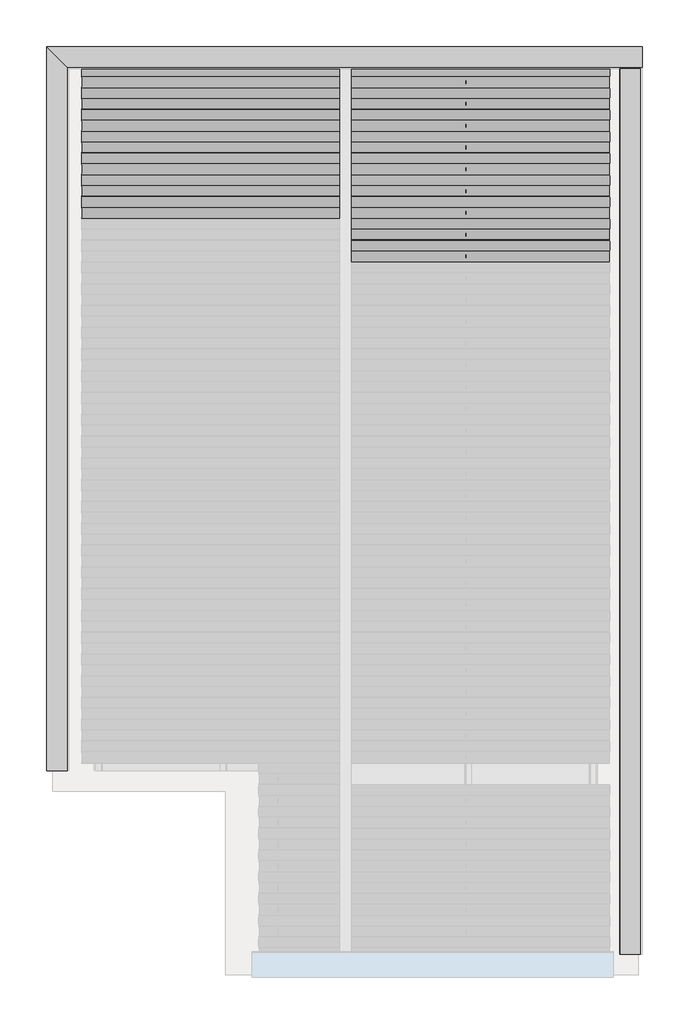
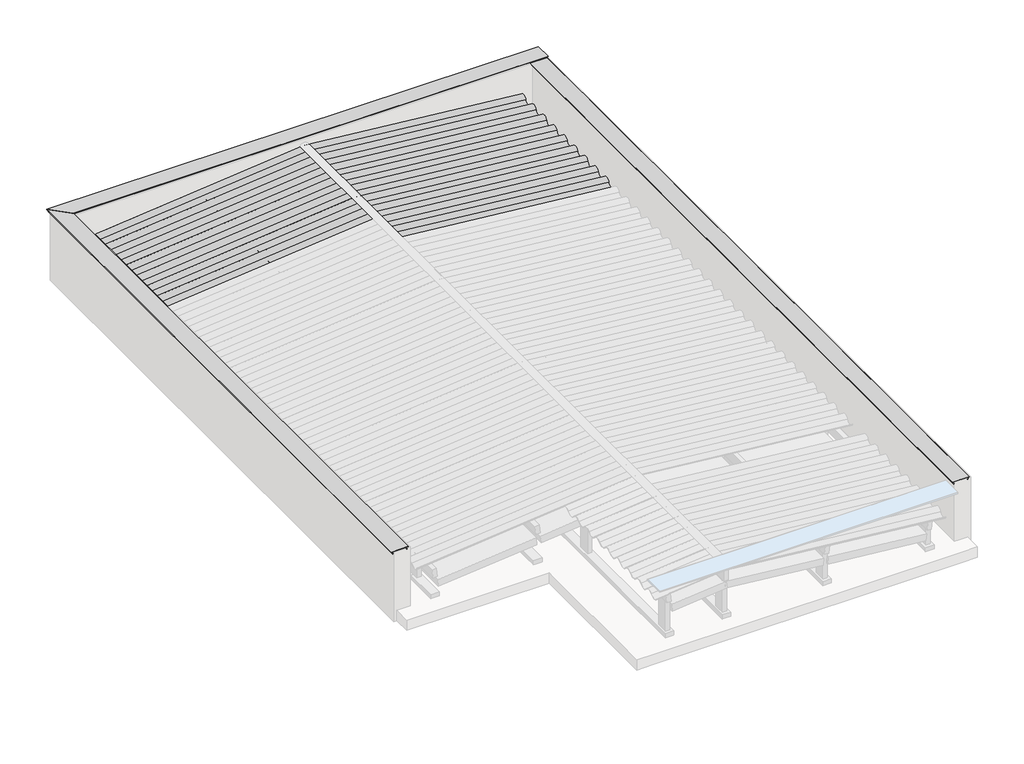
# One storey, part 4 of 4: 23 beams, 10 columns, 1 proxy.
"""IFC4 building model written with IfcOpenShell, lengths in millimetres."""

import ifcopenshell
import ifcopenshell.guid

model = None  # the IFC model being written
_history = None  # IfcOwnerHistory: only IFC2X3 demands one
_inside = {}  # id of a spatial element -> (the spatial element, [elements in it])
_under = {}  # id of a project, library or spatial element -> (it, [spatial elements below it])
_declared = {}  # id of a project -> (the project, [libraries it declares])
_typed = {}  # id of a type object -> (the type object, [elements of that type])
_made_of = {}  # id of a material, layer set ... -> (it, [elements and type objects made of it])


def new_model(schema):
    """Start an empty IFC model of exactly this schema.

    Asked for "IFC4X3", IfcOpenShell would pick the latest addendum, in which some entities
    have other attributes; the version numbers below select the first issue.
    IFC2X3 requires an IfcOwnerHistory on every rooted entity: one is made here for all.
    """
    global model, _history
    if schema == "IFC4X3":
        model = ifcopenshell.file(schema_version=(4, 3, 0, 0))
    else:
        model = ifcopenshell.file(schema=schema)
    _inside.clear()
    _under.clear()
    _declared.clear()
    _typed.clear()
    _made_of.clear()
    _history = None
    if model.schema == "IFC2X3":
        org = make("IfcOrganization", Name="unknown")
        user = make(
            "IfcPersonAndOrganization",
            ThePerson=make("IfcPerson", FamilyName="unknown"),
            TheOrganization=org,
        )
        app = make(
            "IfcApplication",
            ApplicationDeveloper=org,
            Version="unknown",
            ApplicationFullName="unknown",
            ApplicationIdentifier="unknown",
        )
        _history = make(
            "IfcOwnerHistory",
            OwningUser=user,
            OwningApplication=app,
            ChangeAction="ADDED",
            CreationDate=0,
        )
    return model


def make(cls, **values):
    """One entity of the class cls with the attributes given. An attribute that is None is left unset."""
    return model.create_entity(
        cls, **{name: value for name, value in values.items() if value is not None}
    )


def rooted(cls, **values):
    """An entity with a GlobalId (a new one), such as an element, a storey or a relation."""
    return make(cls, GlobalId=ifcopenshell.guid.new(), OwnerHistory=_history, **values)


def si_unit(unit_type, name, prefix=None):
    """IfcSIUnit, for example si_unit("LENGTHUNIT", "METRE", prefix="MILLI")."""
    return make("IfcSIUnit", UnitType=unit_type, Prefix=prefix, Name=name)


def assignment(units):
    """IfcUnitAssignment: the units of a project."""
    return None if units is None else make("IfcUnitAssignment", Units=units)


def point(xyz):
    """IfcCartesianPoint."""
    return None if xyz is None else make("IfcCartesianPoint", Coordinates=xyz)


def direction(xyz):
    """IfcDirection."""
    return None if xyz is None else make("IfcDirection", DirectionRatios=xyz)


def frame(location, z_axis=None, x_axis=None):
    """IfcAxis2Placement3D, a coordinate frame: its origin and axes. An axis left out is left unset."""
    return make(
        "IfcAxis2Placement3D",
        Location=point(location),
        Axis=direction(z_axis),
        RefDirection=direction(x_axis),
    )


def frame_2d(location, x_axis=None):
    """IfcAxis2Placement2D, a coordinate frame in the plane: its origin and x axis."""
    return make(
        "IfcAxis2Placement2D", Location=point(location), RefDirection=direction(x_axis)
    )


def origin():
    """The frame at (0, 0, 0) with its axes left unset."""
    return frame((0.0, 0.0, 0.0))


def place(relative_to, where):
    """IfcLocalPlacement: puts the frame where relative to a parent placement (None: the world)."""
    return make(
        "IfcLocalPlacement", PlacementRelTo=relative_to, RelativePlacement=where
    )


def context(
    kind, dimensions, precision=None, world=None, true_north=None, identifier=None
):
    """IfcGeometricRepresentationContext, for example the 3D "Model" context."""
    return make(
        "IfcGeometricRepresentationContext",
        ContextIdentifier=identifier,
        ContextType=kind,
        CoordinateSpaceDimension=dimensions,
        Precision=precision,
        WorldCoordinateSystem=world,
        TrueNorth=true_north,
    )


def project(units=None, contexts=None):
    """IfcProject with its units and contexts."""
    return rooted(
        "IfcProject",
        Name="project",
        RepresentationContexts=contexts,
        UnitsInContext=assignment(units),
    )


def spatial(cls, under=None, at=None, **own):
    """A site, building, storey or space (cls), placed at a placement, below another one or the project."""
    s = rooted(cls, ObjectPlacement=at, **own)
    if under is not None:
        _under.setdefault(under.id(), (under, []))[1].append(s)
    return s


def polyline(points):
    """IfcPolyline through the points."""
    return make("IfcPolyline", Points=[point(p) for p in points])


def circle_curve(where, radius):
    """IfcCircle in the frame where."""
    return make("IfcCircle", Position=where, Radius=radius)


def ellipse_curve(where, semi_axis1, semi_axis2):
    """IfcEllipse in the frame where."""
    return make(
        "IfcEllipse", Position=where, SemiAxis1=semi_axis1, SemiAxis2=semi_axis2
    )


def trimmed(basis, trim1, trim2, sense, master):
    """IfcTrimmedCurve: the piece of a basis curve between two trims."""
    return make(
        "IfcTrimmedCurve",
        BasisCurve=basis,
        Trim1=trim1,
        Trim2=trim2,
        SenseAgreement=sense,
        MasterRepresentation=master,
    )


def segment(curve, same_sense, transition):
    """IfcCompositeCurveSegment."""
    return make(
        "IfcCompositeCurveSegment",
        Transition=transition,
        SameSense=same_sense,
        ParentCurve=curve,
    )


def composite_curve(segments, self_intersect=None):
    """IfcCompositeCurve: segments joined end to end."""
    return make("IfcCompositeCurve", Segments=segments, SelfIntersect=self_intersect)


def outline(outer, holes=None, kind="AREA"):
    """IfcArbitraryClosedProfileDef: a profile drawn as a closed curve; with holes, ...WithVoids."""
    if holes is None:
        return make("IfcArbitraryClosedProfileDef", ProfileType=kind, OuterCurve=outer)
    return make(
        "IfcArbitraryProfileDefWithVoids",
        ProfileType=kind,
        OuterCurve=outer,
        InnerCurves=holes,
    )


def extrude(swept, where, along, depth):
    """IfcExtrudedAreaSolid: the profile swept, set in the frame where, extruded along a direction by depth."""
    return make(
        "IfcExtrudedAreaSolid",
        SweptArea=swept,
        Position=where,
        ExtrudedDirection=direction(along),
        Depth=depth,
    )


def faces_of(points, faces, orient=None, outer=None):
    """IfcFace entities. A face is a list of loops; a loop is a list of indices into points, from 0.

    orient and outer hold one flag for each loop. By default every Orientation is true, the
    first loop of a face is its IfcFaceOuterBound and the others are IfcFaceBound.
    """
    made = []
    for i, loops in enumerate(faces):
        bounds = []
        for j, loop in enumerate(loops):
            is_outer = j == 0 if outer is None else outer[i][j]
            bounds.append(
                make(
                    "IfcFaceOuterBound" if is_outer else "IfcFaceBound",
                    Bound=make("IfcPolyLoop", Polygon=[points[k] for k in loop]),
                    Orientation=True if orient is None else orient[i][j],
                )
            )
        made.append(make("IfcFace", Bounds=bounds))
    return made


def faceted_brep(points, faces, orient=None, outer=None, voids=None):
    """IfcFacetedBrep: a solid bounded by flat faces; with voids (closed shells), ...WithVoids."""
    shared = [point(p) for p in points]
    hull = make("IfcClosedShell", CfsFaces=faces_of(shared, faces, orient, outer))
    if voids is None:
        return make("IfcFacetedBrep", Outer=hull)
    return make(
        "IfcFacetedBrepWithVoids",
        Outer=hull,
        Voids=[
            make(cls, CfsFaces=faces_of(shared, fs, o, b)) for cls, fs, o, b in voids
        ],
    )


def shape(context_of_items, identifier, shape_type, items):
    """IfcShapeRepresentation: the items that make up one representation, for example the "Body"."""
    return make(
        "IfcShapeRepresentation",
        ContextOfItems=context_of_items,
        RepresentationIdentifier=identifier,
        RepresentationType=shape_type,
        Items=items,
    )


def source(mapping_origin, context_of_items, identifier, shape_type, items):
    """IfcRepresentationMap: a shape defined once, which mapped items show again and again."""
    return make(
        "IfcRepresentationMap",
        MappingOrigin=mapping_origin,
        MappedRepresentation=shape(context_of_items, identifier, shape_type, items),
    )


def transform(
    local_origin,
    x_axis=None,
    y_axis=None,
    z_axis=None,
    scale=None,
    scale2=None,
    scale3=None,
    uniform=True,
):
    """IfcCartesianTransformationOperator3D, or its non-uniform kind. x_axis, y_axis, z_axis: its Axis1, 2, 3."""
    if uniform:
        return make(
            "IfcCartesianTransformationOperator3D",
            Axis1=direction(x_axis),
            Axis2=direction(y_axis),
            LocalOrigin=point(local_origin),
            Scale=scale,
            Axis3=direction(z_axis),
        )
    return make(
        "IfcCartesianTransformationOperator3DnonUniform",
        Axis1=direction(x_axis),
        Axis2=direction(y_axis),
        LocalOrigin=point(local_origin),
        Scale=scale,
        Axis3=direction(z_axis),
        Scale2=scale2,
        Scale3=scale3,
    )


def mapped(mapping_source, mapping_target):
    """IfcMappedItem: shows the shape of a source again, moved by a transform."""
    return make(
        "IfcMappedItem", MappingSource=mapping_source, MappingTarget=mapping_target
    )


def made_of(thing, what):
    """Note that an element or type object is made of a material, layer set ...; save() writes the relation."""
    if what is not None:
        _made_of.setdefault(what.id(), (what, []))[1].append(thing)
    return thing


def element(
    cls,
    number,
    at=None,
    inside=None,
    cuts=None,
    type_object=None,
    material=None,
    context=None,
    identifier="Body",
    shape_type=None,
    held_by="IfcProductDefinitionShape",
    body=None,
    shapes=None,
    **own,
):
    """One element of the class cls, such as IfcWall. Its Tag is "e" and its number.

    at: its placement. inside: the storey or other place that contains it. cuts: it is an
    opening in that element (IfcRelVoidsElement). A single representation is given by context,
    identifier, shape_type and body (its items); several are given by shapes. held_by: the class
    of the entity that holds the representations. save() writes the other relations.
    """
    e = rooted(cls, Tag="e%d" % number, ObjectPlacement=at, **own)
    if body is not None:
        shapes = [shape(context, identifier, shape_type, body)]
    if shapes is not None:
        e.Representation = make(held_by, Representations=shapes)
    if inside is not None:
        _inside.setdefault(inside.id(), (inside, []))[1].append(e)
    if cuts is not None:
        rooted(
            "IfcRelVoidsElement", RelatingBuildingElement=cuts, RelatedOpeningElement=e
        )
    if type_object is not None:
        _typed.setdefault(type_object.id(), (type_object, []))[1].append(e)
    return made_of(e, material)


def aggregate(whole, parts):
    """IfcRelAggregates: a whole, such as a stair, and the parts it consists of."""
    return rooted("IfcRelAggregates", RelatingObject=whole, RelatedObjects=parts)


def save(model, path):
    """Write the relations noted so far, then the file.

    IfcRelAggregates (storeys below a building ...), IfcRelContainedInSpatialStructure (elements
    in a storey), IfcRelDefinesByType, IfcRelAssociatesMaterial and IfcRelDeclares: one each for
    every whole, place, type object, material and project.
    """
    for whole, parts in _under.values():
        aggregate(whole, parts)
    for where, things in _inside.values():
        rooted(
            "IfcRelContainedInSpatialStructure",
            RelatedElements=things,
            RelatingStructure=where,
        )
    for kind, things in _typed.values():
        rooted("IfcRelDefinesByType", RelatedObjects=things, RelatingType=kind)
    for what, things in _made_of.values():
        rooted("IfcRelAssociatesMaterial", RelatedObjects=things, RelatingMaterial=what)
    for by, libraries in _declared.values():
        rooted("IfcRelDeclares", RelatingContext=by, RelatedDefinitions=libraries)
    model.write(path)


def plane_surface(at):
    """IfcPlane: the flat surface through the origin of the frame at, square to its z axis."""
    return make("IfcPlane", Position=at)


def cylinder_surface(at, radius):
    """IfcCylindricalSurface: all points at the distance radius from the z axis of the frame at."""
    return make("IfcCylindricalSurface", Position=at, Radius=radius)


def revolved_surface(curve, axis_point, axis_direction):
    """IfcSurfaceOfRevolution: the curve turned about the line through axis_point along axis_direction."""
    return make(
        "IfcSurfaceOfRevolution",
        SweptCurve=make("IfcArbitraryOpenProfileDef", ProfileType="CURVE", Curve=curve),
        AxisPosition=make("IfcAxis1Placement", Location=point(axis_point), Axis=direction(axis_direction)),
    )


def advanced_brep(points, edges, surfaces, faces):
    """IfcAdvancedBrep: a solid bounded by faces that lie on surfaces and meet in shared edges.

    An edge is (start, end): straight between two places in points (the first is 0);
    or (start, end, curve); or (start, end, curve, False) where it runs against its curve.
    A face is (place in surfaces, loops), or (place, loops, False) where it looks against
    its surface's normal. A loop lists edges by number (the first is 1), with a minus sign
    where the edge is run from its end to its start. The first loop is the outer one.
    """
    corners = [point(p) for p in points]
    vertices = [make("IfcVertexPoint", VertexGeometry=c) for c in corners]
    made = []
    for start, end, *more in edges:
        made.append(
            make(
                "IfcEdgeCurve",
                EdgeStart=vertices[start],
                EdgeEnd=vertices[end],
                EdgeGeometry=more[0] if more else make("IfcPolyline", Points=[corners[start], corners[end]]),
                SameSense=more[1] if len(more) > 1 else True,
            )
        )
    hull = []
    for where, loops, *sense in faces:
        bounds = []
        for j, loop in enumerate(loops):
            ring = [make("IfcOrientedEdge", EdgeElement=made[abs(k) - 1], Orientation=k > 0) for k in loop]
            bounds.append(
                make(
                    "IfcFaceOuterBound" if j == 0 else "IfcFaceBound",
                    Bound=make("IfcEdgeLoop", EdgeList=ring),
                    Orientation=True,
                )
            )
        hull.append(make("IfcAdvancedFace", Bounds=bounds, FaceSurface=surfaces[where], SameSense=sense[0] if sense else True))
    return make("IfcAdvancedBrep", Outer=make("IfcClosedShell", CfsFaces=hull))


def column_7d6827b5(model_context):
    return source(origin(), model_context, "Body", "SweptSolid", [
        extrude(outline(polyline([(30.0, 80.0), (30.0, -80.0), (-30.0, -80.0), (-30.0, 80.0), (30.0, 80.0)])), frame((0.0, 0.0, 4460.0), z_axis=(0.0, 0.0, 1.0), x_axis=(1.0, 0.0, 0.0)), (0.0, 0.0, 1.0), 466.0),
    ])


def column_c7348c99(model_context):
    return source(origin(), model_context, "Body", "SweptSolid", [
        extrude(outline(polyline([(30.0, 80.0), (30.0, -80.0), (-30.0, -80.0), (-30.0, 80.0), (30.0, 80.0)])), frame((0.0, 0.0, 4460.0), z_axis=(0.0, 0.0, 1.0), x_axis=(1.0, 0.0, 0.0)), (0.0, 0.0, 1.0), 372.8),
    ])


def column_6cc9e01b(model_context):
    return source(origin(), model_context, "Body", "SweptSolid", [
        extrude(outline(polyline([(30.0, 80.0), (30.0, -80.0), (-30.0, -80.0), (-30.0, 80.0), (30.0, 80.0)])), frame((0.0, 0.0, 4460.0), z_axis=(0.0, 0.0, 1.0), x_axis=(1.0, 0.0, 0.0)), (0.0, 0.0, 1.0), 233.0),
    ])


model = new_model("IFC4")

# Units and contexts
model_context = context("Model", 3, world=origin())
ifc_project = project(units=[si_unit("LENGTHUNIT", "METRE", prefix="MILLI")], contexts=[model_context])

# Site, building, storey
site = spatial("IfcSite", under=ifc_project)
building = spatial("IfcBuilding", under=site)
storey = spatial("IfcBuildingStorey", under=building, Name="COB. SALA ESTAR", Elevation=4400.0)

# Beams
placement = place(None, origin())
element("IfcBeam", 1, ObjectType="Madeira de lei : Berço 6x12cm", at=placement, inside=storey, context=model_context, shape_type="SweptSolid", body=[
    extrude(outline(polyline([(-3400.8557491, 5593.4722664), (-3280.8557491, 5593.4722664), (-3280.8557491, 4180.4300153), (-3400.8557491, 4180.4300153), (-3400.8557491, 5593.4722664)])), frame((0.0, 0.0, 4400.0), z_axis=(0.0, 0.0, 1.0), x_axis=(1.0, 0.0, 0.0)), (0.0, 0.0, 1.0), 60.0),
])
element("IfcBeam", 2, ObjectType="Madeira de lei : Berço 6x12cm", at=placement, inside=storey, context=model_context, shape_type="SweptSolid", body=[
    extrude(outline(polyline([(-2032.3324227, 4180.4300153), (-1912.3324227, 4180.4300153), (-1912.3324227, 2180.4300159), (-2032.3324227, 2180.4300159), (-2032.3324227, 4180.4300153)])), frame((0.0, 0.0, 4400.0), z_axis=(0.0, 0.0, 1.0), x_axis=(1.0, 0.0, 0.0)), (0.0, 0.0, 1.0), 60.0),
])
element("IfcBeam", 3, ObjectType="Madeira de lei : Berço 6x12cm", at=placement, inside=storey, context=model_context, shape_type="SweptSolid", body=[
    extrude(outline(polyline([(-2032.3324227, 5593.4722664), (-1912.3324227, 5593.4722664), (-1912.3324227, 4180.4300153), (-2032.3324227, 4180.4300153), (-2032.3324227, 5593.4722664)])), frame((0.0, 0.0, 4400.0), z_axis=(0.0, 0.0, 1.0), x_axis=(1.0, 0.0, 0.0)), (0.0, 0.0, 1.0), 60.0),
])
element("IfcBeam", 4, ObjectType="Madeira de lei : Berço 6x12cm", at=placement, inside=storey, context=model_context, shape_type="SweptSolid", body=[
    extrude(outline(polyline([(-634.0324227, 4180.4300153), (-514.0324227, 4180.4300153), (-514.0324227, 2180.4300159), (-634.0324227, 2180.4300159), (-634.0324227, 4180.4300153)])), frame((0.0, 0.0, 4400.0), z_axis=(0.0, 0.0, 1.0), x_axis=(1.0, 0.0, 0.0)), (0.0, 0.0, 1.0), 60.0),
])
element("IfcBeam", 5, ObjectType="Madeira de lei : Berço 6x12cm", at=placement, inside=storey, context=model_context, shape_type="SweptSolid", body=[
    extrude(outline(polyline([(-634.0324227, 5593.4722664), (-514.0324227, 5593.4722664), (-514.0324227, 4180.4300153), (-634.0324227, 4180.4300153), (-634.0324227, 5593.4722664)])), frame((0.0, 0.0, 4400.0), z_axis=(0.0, 0.0, 1.0), x_axis=(1.0, 0.0, 0.0)), (0.0, 0.0, 1.0), 60.0),
])
element("IfcBeam", 6, ObjectType="Madeira de lei : Berço 6x12cm", at=placement, inside=storey, context=model_context, shape_type="SweptSolid", body=[
    extrude(outline(polyline([(-6167.5301913, 5593.4722664), (-6047.5301913, 5593.4722664), (-6047.5301913, 4180.4300153), (-6167.5301913, 4180.4300153), (-6167.5301913, 5593.4722664)])), frame((0.0, 0.0, 4400.0), z_axis=(0.0, 0.0, 1.0), x_axis=(1.0, 0.0, 0.0)), (0.0, 0.0, 1.0), 60.0),
])
element("IfcBeam", 7, ObjectType="Madeira de lei : Berço 6x12cm", at=placement, inside=storey, context=model_context, shape_type="SweptSolid", body=[
    extrude(outline(polyline([(-4769.2301913, 5593.4722664), (-4649.2301913, 5593.4722664), (-4649.2301913, 4180.4300153), (-4769.2301913, 4180.4300153), (-4769.2301913, 5593.4722664)])), frame((0.0, 0.0, 4400.0), z_axis=(0.0, 0.0, 1.0), x_axis=(1.0, 0.0, 0.0)), (0.0, 0.0, 1.0), 60.0),
])
element("IfcBeam", 8, ObjectType="Telha Ondulada : Fibrocimento", at=placement, inside=storey, context=model_context, shape_type="SweptSolid", body=[
    extrude(outline(composite_curve([segment(trimmed(circle_curve(frame_2d((-58.7002978, -53.2060538)), 66.7939461), [point((-29.3501489, 6.7939462))], [point((-29.3501489, -113.2060538))], False, "CARTESIAN"), True, "CONTINUOUS"), segment(polyline([(-29.3501489, -113.2060538), (-31.5472154, -108.7146288)]), True, "CONTINUOUS"), segment(trimmed(circle_curve(frame_2d((-58.7002978, -53.2060538)), 61.7939461), [point((-31.5472154, -108.7146288))], [point((-31.5472154, 2.3025211))], True, "CARTESIAN"), True, "CONTINUOUS"), segment(trimmed(circle_curve(frame_2d((0.0, 66.7939462)), 71.7939461), [point((-31.5472154, 2.3025211))], [point((-31.5472154, 131.2853712))], False, "CARTESIAN"), True, "CONTINUOUS"), segment(polyline([(-31.5472154, 131.2853712), (-29.3501489, 126.7939462)]), True, "CONTINUOUS"), segment(trimmed(circle_curve(frame_2d((0.0, 66.7939462)), 66.7939461), [point((-29.3501489, 126.7939462))], [point((-29.3501489, 6.7939462))], True, "CARTESIAN"), True, "CONTINUOUS")], self_intersect=False)), frame((-6307.6707245, 4045.326948, 4862.7215886), z_axis=(0.9950371902099892, 0.0, 0.09950371902099954), x_axis=(-0.09950371902099954, 0.0, 0.9950371902099892)), (0.0, 0.0, 1.0), 2972.5075682),
])
element("IfcBeam", 9, ObjectType="Telha Ondulada : Fibrocimento", at=placement, inside=storey, context=model_context, shape_type="SweptSolid", body=[
    extrude(outline(composite_curve([segment(trimmed(circle_curve(frame_2d((-58.7002978, -53.2060538)), 66.7939461), [point((-29.3501489, 6.7939462))], [point((-29.3501489, -113.2060538))], False, "CARTESIAN"), True, "CONTINUOUS"), segment(polyline([(-29.3501489, -113.2060538), (-31.5472154, -108.7146288)]), True, "CONTINUOUS"), segment(trimmed(circle_curve(frame_2d((-58.7002978, -53.2060538)), 61.7939461), [point((-31.5472154, -108.7146288))], [point((-31.5472154, 2.3025211))], True, "CARTESIAN"), True, "CONTINUOUS"), segment(trimmed(circle_curve(frame_2d((0.0, 66.7939462)), 71.7939461), [point((-31.5472154, 2.3025211))], [point((-31.5472154, 131.2853712))], False, "CARTESIAN"), True, "CONTINUOUS"), segment(polyline([(-31.5472154, 131.2853712), (-29.3501489, 126.7939462)]), True, "CONTINUOUS"), segment(trimmed(circle_curve(frame_2d((0.0, 66.7939462)), 66.7939461), [point((-29.3501489, 126.7939462))], [point((-29.3501489, 6.7939462))], True, "CARTESIAN"), True, "CONTINUOUS")], self_intersect=False)), frame((-6307.6707245, 4289.826948, 4862.7215886), z_axis=(0.9950371902099892, 0.0, 0.09950371902099969), x_axis=(-0.09950371902099969, 0.0, 0.9950371902099892)), (0.0, 0.0, 1.0), 2972.5075682),
])
element("IfcBeam", 10, ObjectType="Telha Ondulada : Fibrocimento", at=placement, inside=storey, context=model_context, shape_type="SweptSolid", body=[
    extrude(outline(composite_curve([segment(trimmed(circle_curve(frame_2d((-58.7002978, -53.2060538)), 66.7939461), [point((-29.3501489, 6.7939462))], [point((-29.3501489, -113.2060538))], False, "CARTESIAN"), True, "CONTINUOUS"), segment(polyline([(-29.3501489, -113.2060538), (-31.5472154, -108.7146288)]), True, "CONTINUOUS"), segment(trimmed(circle_curve(frame_2d((-58.7002978, -53.2060538)), 61.7939461), [point((-31.5472154, -108.7146288))], [point((-31.5472154, 2.3025211))], True, "CARTESIAN"), True, "CONTINUOUS"), segment(trimmed(circle_curve(frame_2d((0.0, 66.7939462)), 71.7939461), [point((-31.5472154, 2.3025211))], [point((-31.5472154, 131.2853712))], False, "CARTESIAN"), True, "CONTINUOUS"), segment(polyline([(-31.5472154, 131.2853712), (-29.3501489, 126.7939462)]), True, "CONTINUOUS"), segment(trimmed(circle_curve(frame_2d((0.0, 66.7939462)), 66.7939461), [point((-29.3501489, 126.7939462))], [point((-29.3501489, 6.7939462))], True, "CARTESIAN"), True, "CONTINUOUS")], self_intersect=False)), frame((-6307.6707245, 4534.326948, 4862.7215886), z_axis=(0.9950371902099892, 0.0, 0.09950371902099972), x_axis=(-0.09950371902099972, 0.0, 0.9950371902099892)), (0.0, 0.0, 1.0), 2972.5075682),
])
element("IfcBeam", 11, ObjectType="Telha Ondulada : Fibrocimento", at=placement, inside=storey, context=model_context, shape_type="SweptSolid", body=[
    extrude(outline(composite_curve([segment(trimmed(circle_curve(frame_2d((-58.7002978, -53.2060538)), 66.7939461), [point((-29.3501489, 6.7939462))], [point((-29.3501489, -113.2060538))], False, "CARTESIAN"), True, "CONTINUOUS"), segment(polyline([(-29.3501489, -113.2060538), (-31.5472154, -108.7146288)]), True, "CONTINUOUS"), segment(trimmed(circle_curve(frame_2d((-58.7002978, -53.2060538)), 61.7939461), [point((-31.5472154, -108.7146288))], [point((-31.5472154, 2.3025211))], True, "CARTESIAN"), True, "CONTINUOUS"), segment(trimmed(circle_curve(frame_2d((0.0, 66.7939462)), 71.7939461), [point((-31.5472154, 2.3025211))], [point((-31.5472154, 131.2853712))], False, "CARTESIAN"), True, "CONTINUOUS"), segment(polyline([(-31.5472154, 131.2853712), (-29.3501489, 126.7939462)]), True, "CONTINUOUS"), segment(trimmed(circle_curve(frame_2d((0.0, 66.7939462)), 66.7939461), [point((-29.3501489, 126.7939462))], [point((-29.3501489, 6.7939462))], True, "CARTESIAN"), True, "CONTINUOUS")], self_intersect=False)), frame((-6307.6707245, 4778.826948, 4862.7215886), z_axis=(0.9950371902099892, 0.0, 0.09950371902099972), x_axis=(-0.09950371902099972, 0.0, 0.9950371902099892)), (0.0, 0.0, 1.0), 2972.5075682),
])
element("IfcBeam", 12, ObjectType="Telha Ondulada : Fibrocimento", at=placement, inside=storey, context=model_context, shape_type="SweptSolid", body=[
    extrude(outline(composite_curve([segment(trimmed(circle_curve(frame_2d((-58.7002978, -53.2060538)), 66.7939461), [point((-29.3501489, 6.7939462))], [point((-29.3501489, -113.2060538))], False, "CARTESIAN"), True, "CONTINUOUS"), segment(polyline([(-29.3501489, -113.2060538), (-31.5472154, -108.7146288)]), True, "CONTINUOUS"), segment(trimmed(circle_curve(frame_2d((-58.7002978, -53.2060538)), 61.7939461), [point((-31.5472154, -108.7146288))], [point((-31.5472154, 2.3025211))], True, "CARTESIAN"), True, "CONTINUOUS"), segment(trimmed(circle_curve(frame_2d((0.0, 66.7939462)), 71.7939461), [point((-31.5472154, 2.3025211))], [point((-31.5472154, 131.2853712))], False, "CARTESIAN"), True, "CONTINUOUS"), segment(polyline([(-31.5472154, 131.2853712), (-29.3501489, 126.7939462)]), True, "CONTINUOUS"), segment(trimmed(circle_curve(frame_2d((0.0, 66.7939462)), 66.7939461), [point((-29.3501489, 126.7939462))], [point((-29.3501489, 6.7939462))], True, "CARTESIAN"), True, "CONTINUOUS")], self_intersect=False)), frame((-6307.6707245, 5023.326948, 4862.7215886), z_axis=(0.9950371902099892, 0.0, 0.09950371902099968), x_axis=(-0.09950371902099968, 0.0, 0.9950371902099892)), (0.0, 0.0, 1.0), 2972.5075682),
])
element("IfcBeam", 13, ObjectType="Telha Ondulada : Fibrocimento", at=placement, inside=storey, context=model_context, shape_type="SweptSolid", body=[
    extrude(outline(composite_curve([segment(trimmed(circle_curve(frame_2d((-58.7002978, -53.2060538)), 66.7939461), [point((-29.3501489, 6.7939462))], [point((-29.3501489, -113.2060538))], False, "CARTESIAN"), True, "CONTINUOUS"), segment(polyline([(-29.3501489, -113.2060538), (-31.5472154, -108.7146288)]), True, "CONTINUOUS"), segment(trimmed(circle_curve(frame_2d((-58.7002978, -53.2060538)), 61.7939461), [point((-31.5472154, -108.7146288))], [point((-31.5472154, 2.3025211))], True, "CARTESIAN"), True, "CONTINUOUS"), segment(trimmed(circle_curve(frame_2d((0.0, 66.7939462)), 71.7939461), [point((-31.5472154, 2.3025211))], [point((-31.5472154, 131.2853712))], False, "CARTESIAN"), True, "CONTINUOUS"), segment(polyline([(-31.5472154, 131.2853712), (-29.3501489, 126.7939462)]), True, "CONTINUOUS"), segment(trimmed(circle_curve(frame_2d((0.0, 66.7939462)), 66.7939461), [point((-29.3501489, 126.7939462))], [point((-29.3501489, 6.7939462))], True, "CARTESIAN"), True, "CONTINUOUS")], self_intersect=False)), frame((-6307.6707245, 5267.826948, 4862.7215886), z_axis=(0.9950371902099892, 0.0, 0.09950371902099968), x_axis=(-0.09950371902099968, 0.0, 0.9950371902099892)), (0.0, 0.0, 1.0), 2972.5075682),
])
element("IfcBeam", 14, ObjectType="Telha Ondulada : Fibrocimento", at=placement, inside=storey, context=model_context, shape_type="AdvancedBrep", body=[
    advanced_brep(
    [(-3346.994697, 5505.5330018, 5129.2926567), (-3346.994697, 5385.5330018, 5129.2926567), (-3346.7760807, 5381.0415768, 5127.1064938), (-3346.7760807, 5510.0244269, 5127.1064938), (-3346.7760807, 5621.0415768, 5127.1064938), (-3346.994697, 5625.5330018, 5129.2926567), (-6304.5316593, 5510.0244269, 4831.330936), (-6304.5316593, 5381.0415768, 4831.330936), (-6304.7502755, 5385.5330018, 4833.5170989), (-6304.7502755, 5505.5330018, 4833.5170989), (-6306.3985657, 5614.0430027, 4850.0), (-6306.3985657, 5606.8885423, 4850.0), (-6230.281307, 5613.9936641, 4850.0), (-6230.281307, 5621.0415768, 4838.7559712), (-6117.841019, 5621.0415768, 4850.0), (-6230.281307, 5625.5330018, 4840.9639958), (-6139.9212645, 5625.5330018, 4850.0), (-6230.281307, 5620.2264681, 4850.0)],
    [
        (0, 1, circle_curve(frame((-3349.915146, 5445.5330018, 5158.4971465), z_axis=(-0.9950371902099892, 0.0, -0.09950371902099951), x_axis=(0.0893826983688464, -0.43941330938261886, -0.8938269836885206)), 66.7939461)),
        (1, 2),
        (2, 3, circle_curve(frame((-3349.915146, 5445.5330018, 5158.4971465), z_axis=(0.9950371902099892, 0.0, 0.09950371902099951), x_axis=(0.08938269836885925, 0.4394133093826069, -0.8938269836885252)), 71.7939461)),
        (3, 4, circle_curve(frame((-3344.074248, 5565.5330018, 5100.088167), z_axis=(-0.9950371902099892, 0.0, -0.09950371902099951), x_axis=(-0.0893826983688466, 0.4394133093826145, 0.8938269836885228)), 61.7939461)),
        (4, 5),
        (5, 0, circle_curve(frame((-3344.074248, 5565.5330018, 5100.088167), z_axis=(0.9950371902099892, 0.0, 0.09950371902099951), x_axis=(-0.08938269836885811, -0.4394133093826303, 0.8938269836885137)), 66.7939461)),
        (6, 7, circle_curve(frame((-6307.6707245, 5445.5330018, 4862.7215886), z_axis=(-0.9950371902099892, 0.0, -0.09950371902099951), x_axis=(0.08938269836885925, 0.4394133093826069, -0.8938269836885252)), 71.7939461)),
        (7, 8),
        (8, 9, circle_curve(frame((-6307.6707245, 5445.5330018, 4862.7215886), z_axis=(0.9950371902099892, 0.0, 0.09950371902099951), x_axis=(0.0893826983688464, -0.43941330938261886, -0.8938269836885206)), 66.7939461)),
        (9, 10, circle_curve(frame((-6301.8298266, 5565.5330018, 4804.3126092), z_axis=(-0.9950371902099892, 0.0, -0.09950371902099951), x_axis=(-0.08938269836885811, -0.4394133093826303, 0.8938269836885137)), 66.7939461)),
        (10, 11),
        (11, 6, circle_curve(frame((-6301.8298266, 5565.5330018, 4804.3126092), z_axis=(0.9950371902099892, 0.0, 0.09950371902099951), x_axis=(-0.0893826983688466, 0.4394133093826145, 0.8938269836885228)), 61.7939461)),
        (0, 9),
        (8, 1),
        (7, 2),
        (6, 3),
        (11, 12, ellipse_curve(frame((-5844.9559183, 5565.5330018, 4850.0), z_axis=(0.0, 0.0, -1.0), x_axis=(-0.9999999999999999, 0.0, 0.0)), 621.0214729, 61.7939461)),
        (12, 13, ellipse_curve(frame((-6230.281307, 5565.5330018, 4811.4674611), z_axis=(-1.0, 0.0, 0.0), x_axis=(0.0, 0.0, -1.0)), 62.1021473, 61.7939461)),
        (13, 14),
        (14, 4),
        (13, 15),
        (15, 16),
        (16, 5),
        (15, 17, ellipse_curve(frame((-6230.281307, 5565.5330018, 4811.4674611), z_axis=(1.0, 0.0, 0.0), x_axis=(0.0, 0.0, -1.0)), 67.1270851, 66.7939461)),
        (17, 10, ellipse_curve(frame((-5844.9559183, 5565.5330018, 4850.0), z_axis=(0.0, 0.0, 1.0), x_axis=(-0.9999999999999999, 0.0, 0.0)), 671.270851, 66.7939461)),
        (12, 17),
    ],
    [
        plane_surface(frame((-3349.915146, 5512.326948, 5158.4971465), z_axis=(0.9950371902099892, 0.0, 0.09950371902099951), x_axis=(0.09950371902099951, 0.0, -0.9950371902099892))),
        plane_surface(frame((-6307.6707245, 5512.326948, 4862.7215886), z_axis=(-0.9950371902099892, 0.0, -0.09950371902099951), x_axis=(-0.09950371902099951, 0.0, 0.9950371902099892))),
        revolved_surface(polyline([(-6301.70050136783, 5416.182852897475, 4803.019357278286), (-3343.9449228430767, 5416.182852897475, 5098.794915130763)]), (-3349.915146, 5445.5330018, 5158.4971465), (-0.9950371902099892, 0.0, -0.09950371902099951)),
        plane_surface(frame((-3346.8853889, 5383.2872893, 5128.1995753), z_axis=(-0.08938269836883676, -0.43941330938305423, 0.8938269836883075), x_axis=(0.04372325847092788, -0.8982850012869147, -0.437232584709388))),
        cylinder_surface(frame((-3349.915146, 5445.5330018, 5158.4971465), z_axis=(-0.9950371902099892, 0.0, -0.09950371902099951), x_axis=(0.08938269836885925, 0.4394133093826069, -0.8938269836885252)), 71.7939461),
        revolved_surface(polyline([(-6465.351973387851, 5592.686084155613, 4843.745821878515), (-3349.597557645277, 5592.686084155613, 5155.3212634527745)]), (-3344.074248, 5565.5330018, 5100.088167), (-0.9950371902099892, 0.0, -0.09950371902099951)),
        plane_surface(frame((-3346.8853889, 5623.2872893, 5128.1995753), z_axis=(0.08938269836887112, 0.4394133093823482, -0.8938269836886512), x_axis=(-0.043723258470857625, 0.8982850012872601, 0.4372325847086854))),
        cylinder_surface(frame((-3344.074248, 5565.5330018, 5100.088167), z_axis=(-0.9950371902099892, 0.0, -0.09950371902099951), x_axis=(-0.08938269836885811, -0.4394133093826303, 0.8938269836885137)), 66.7939461),
        plane_surface(frame((-6230.281307, 5584.4300153, 4850.0), z_axis=(-1.0, 0.0, 0.0), x_axis=(0.0, 0.0, -1.0))),
        plane_surface(frame((-6630.281307, 5584.4300153, 4850.0), z_axis=(0.0, 0.0, -1.0), x_axis=(0.0, -1.0, 0.0))),
    ],
    [
        (0, [[1, 2, 3, 4, 5, 6]]),
        (1, [[7, 8, 9, 10, 11, 12]]),
        (2, [[-1, 13, -9, 14]]),
        (3, [[-2, -14, -8, 15]]),
        (4, [[-3, -15, -7, 16]]),
        (5, [[-4, -16, -12, 17, 18, 19, 20]]),
        (6, [[-5, -20, -19, 21, 22, 23]]),
        (7, [[-6, -23, -22, 24, 25, -10, -13]]),
        (8, [[26, -24, -21, -18]]),
        (9, [[-26, -17, -11, -25]]),
    ],
),
])
element("IfcBeam", 15, ObjectType="Telha Ondulada : Fibrocimento", at=placement, inside=storey, context=model_context, shape_type="SweptSolid", body=[
    extrude(outline(composite_curve([segment(trimmed(circle_curve(frame_2d((0.0, 66.7939462)), 66.7939461), [point((29.3501489, 6.7939462))], [point((29.3501489, 126.7939462))], True, "CARTESIAN"), True, "CONTINUOUS"), segment(polyline([(29.3501489, 126.7939462), (31.5472154, 131.2853712)]), True, "CONTINUOUS"), segment(trimmed(circle_curve(frame_2d((0.0, 66.7939462)), 71.7939461), [point((31.5472154, 131.2853712))], [point((31.5472154, 2.3025211))], False, "CARTESIAN"), True, "CONTINUOUS"), segment(trimmed(circle_curve(frame_2d((58.7002978, -53.2060538)), 61.7939461), [point((31.5472154, 2.3025211))], [point((31.5472154, -108.7146288))], True, "CARTESIAN"), True, "CONTINUOUS"), segment(polyline([(31.5472154, -108.7146288), (29.3501489, -113.2060538)]), True, "CONTINUOUS"), segment(trimmed(circle_curve(frame_2d((58.7002978, -53.2060538)), 66.7939461), [point((29.3501489, -113.2060538))], [point((29.3501489, 6.7939462))], False, "CARTESIAN"), True, "CONTINUOUS")], self_intersect=False)), frame((-373.8918894, 3556.326948, 4862.7215886), z_axis=(-0.9950371902099892, 0.0, 0.09950371902099946), x_axis=(-0.09950371902099946, 0.0, -0.9950371902099892)), (0.0, 0.0, 1.0), 2972.5075682),
])
element("IfcBeam", 16, ObjectType="Telha Ondulada : Fibrocimento", at=placement, inside=storey, context=model_context, shape_type="SweptSolid", body=[
    extrude(outline(composite_curve([segment(trimmed(circle_curve(frame_2d((0.0, 66.7939462)), 66.7939461), [point((29.3501489, 6.7939462))], [point((29.3501489, 126.7939462))], True, "CARTESIAN"), True, "CONTINUOUS"), segment(polyline([(29.3501489, 126.7939462), (31.5472154, 131.2853712)]), True, "CONTINUOUS"), segment(trimmed(circle_curve(frame_2d((0.0, 66.7939462)), 71.7939461), [point((31.5472154, 131.2853712))], [point((31.5472154, 2.3025211))], False, "CARTESIAN"), True, "CONTINUOUS"), segment(trimmed(circle_curve(frame_2d((58.7002978, -53.2060538)), 61.7939461), [point((31.5472154, 2.3025211))], [point((31.5472154, -108.7146288))], True, "CARTESIAN"), True, "CONTINUOUS"), segment(polyline([(31.5472154, -108.7146288), (29.3501489, -113.2060538)]), True, "CONTINUOUS"), segment(trimmed(circle_curve(frame_2d((58.7002978, -53.2060538)), 66.7939461), [point((29.3501489, -113.2060538))], [point((29.3501489, 6.7939462))], False, "CARTESIAN"), True, "CONTINUOUS")], self_intersect=False)), frame((-373.8918894, 3800.826948, 4862.7215886), z_axis=(-0.9950371902099892, 0.0, 0.09950371902099946), x_axis=(-0.09950371902099946, 0.0, -0.9950371902099892)), (0.0, 0.0, 1.0), 2972.5075682),
])
element("IfcBeam", 17, ObjectType="Telha Ondulada : Fibrocimento", at=placement, inside=storey, context=model_context, shape_type="SweptSolid", body=[
    extrude(outline(composite_curve([segment(trimmed(circle_curve(frame_2d((0.0, 66.7939462)), 66.7939461), [point((29.3501489, 6.7939462))], [point((29.3501489, 126.7939462))], True, "CARTESIAN"), True, "CONTINUOUS"), segment(polyline([(29.3501489, 126.7939462), (31.5472154, 131.2853712)]), True, "CONTINUOUS"), segment(trimmed(circle_curve(frame_2d((0.0, 66.7939462)), 71.7939461), [point((31.5472154, 131.2853712))], [point((31.5472154, 2.3025211))], False, "CARTESIAN"), True, "CONTINUOUS"), segment(trimmed(circle_curve(frame_2d((58.7002978, -53.2060538)), 61.7939461), [point((31.5472154, 2.3025211))], [point((31.5472154, -108.7146288))], True, "CARTESIAN"), True, "CONTINUOUS"), segment(polyline([(31.5472154, -108.7146288), (29.3501489, -113.2060538)]), True, "CONTINUOUS"), segment(trimmed(circle_curve(frame_2d((58.7002978, -53.2060538)), 66.7939461), [point((29.3501489, -113.2060538))], [point((29.3501489, 6.7939462))], False, "CARTESIAN"), True, "CONTINUOUS")], self_intersect=False)), frame((-373.8918894, 4045.326948, 4862.7215886), z_axis=(-0.9950371902099892, 0.0, 0.09950371902099946), x_axis=(-0.09950371902099946, 0.0, -0.9950371902099892)), (0.0, 0.0, 1.0), 2972.5075682),
])
element("IfcBeam", 18, ObjectType="Telha Ondulada : Fibrocimento", at=placement, inside=storey, context=model_context, shape_type="SweptSolid", body=[
    extrude(outline(composite_curve([segment(trimmed(circle_curve(frame_2d((0.0, 66.7939462)), 66.7939461), [point((29.3501489, 6.7939462))], [point((29.3501489, 126.7939462))], True, "CARTESIAN"), True, "CONTINUOUS"), segment(polyline([(29.3501489, 126.7939462), (31.5472154, 131.2853712)]), True, "CONTINUOUS"), segment(trimmed(circle_curve(frame_2d((0.0, 66.7939462)), 71.7939461), [point((31.5472154, 131.2853712))], [point((31.5472154, 2.3025211))], False, "CARTESIAN"), True, "CONTINUOUS"), segment(trimmed(circle_curve(frame_2d((58.7002978, -53.2060538)), 61.7939461), [point((31.5472154, 2.3025211))], [point((31.5472154, -108.7146288))], True, "CARTESIAN"), True, "CONTINUOUS"), segment(polyline([(31.5472154, -108.7146288), (29.3501489, -113.2060538)]), True, "CONTINUOUS"), segment(trimmed(circle_curve(frame_2d((58.7002978, -53.2060538)), 66.7939461), [point((29.3501489, -113.2060538))], [point((29.3501489, 6.7939462))], False, "CARTESIAN"), True, "CONTINUOUS")], self_intersect=False)), frame((-373.8918894, 4289.826948, 4862.7215886), z_axis=(-0.9950371902099892, 0.0, 0.09950371902099946), x_axis=(-0.09950371902099946, 0.0, -0.9950371902099892)), (0.0, 0.0, 1.0), 2972.5075682),
])
element("IfcBeam", 19, ObjectType="Telha Ondulada : Fibrocimento", at=placement, inside=storey, context=model_context, shape_type="SweptSolid", body=[
    extrude(outline(composite_curve([segment(trimmed(circle_curve(frame_2d((0.0, 66.7939462)), 66.7939461), [point((29.3501489, 6.7939462))], [point((29.3501489, 126.7939462))], True, "CARTESIAN"), True, "CONTINUOUS"), segment(polyline([(29.3501489, 126.7939462), (31.5472154, 131.2853712)]), True, "CONTINUOUS"), segment(trimmed(circle_curve(frame_2d((0.0, 66.7939462)), 71.7939461), [point((31.5472154, 131.2853712))], [point((31.5472154, 2.3025211))], False, "CARTESIAN"), True, "CONTINUOUS"), segment(trimmed(circle_curve(frame_2d((58.7002978, -53.2060538)), 61.7939461), [point((31.5472154, 2.3025211))], [point((31.5472154, -108.7146288))], True, "CARTESIAN"), True, "CONTINUOUS"), segment(polyline([(31.5472154, -108.7146288), (29.3501489, -113.2060538)]), True, "CONTINUOUS"), segment(trimmed(circle_curve(frame_2d((58.7002978, -53.2060538)), 66.7939461), [point((29.3501489, -113.2060538))], [point((29.3501489, 6.7939462))], False, "CARTESIAN"), True, "CONTINUOUS")], self_intersect=False)), frame((-373.8918894, 4534.326948, 4862.7215886), z_axis=(-0.9950371902099892, 0.0, 0.09950371902099946), x_axis=(-0.09950371902099946, 0.0, -0.9950371902099892)), (0.0, 0.0, 1.0), 2972.5075682),
])
element("IfcBeam", 20, ObjectType="Telha Ondulada : Fibrocimento", at=placement, inside=storey, context=model_context, shape_type="SweptSolid", body=[
    extrude(outline(composite_curve([segment(trimmed(circle_curve(frame_2d((0.0, 66.7939462)), 66.7939461), [point((29.3501489, 6.7939462))], [point((29.3501489, 126.7939462))], True, "CARTESIAN"), True, "CONTINUOUS"), segment(polyline([(29.3501489, 126.7939462), (31.5472154, 131.2853712)]), True, "CONTINUOUS"), segment(trimmed(circle_curve(frame_2d((0.0, 66.7939462)), 71.7939461), [point((31.5472154, 131.2853712))], [point((31.5472154, 2.3025211))], False, "CARTESIAN"), True, "CONTINUOUS"), segment(trimmed(circle_curve(frame_2d((58.7002978, -53.2060538)), 61.7939461), [point((31.5472154, 2.3025211))], [point((31.5472154, -108.7146288))], True, "CARTESIAN"), True, "CONTINUOUS"), segment(polyline([(31.5472154, -108.7146288), (29.3501489, -113.2060538)]), True, "CONTINUOUS"), segment(trimmed(circle_curve(frame_2d((58.7002978, -53.2060538)), 66.7939461), [point((29.3501489, -113.2060538))], [point((29.3501489, 6.7939462))], False, "CARTESIAN"), True, "CONTINUOUS")], self_intersect=False)), frame((-373.8918894, 4778.826948, 4862.7215886), z_axis=(-0.9950371902099892, 0.0, 0.09950371902099946), x_axis=(-0.09950371902099946, 0.0, -0.9950371902099892)), (0.0, 0.0, 1.0), 2972.5075682),
])
element("IfcBeam", 21, ObjectType="Telha Ondulada : Fibrocimento", at=placement, inside=storey, context=model_context, shape_type="SweptSolid", body=[
    extrude(outline(composite_curve([segment(trimmed(circle_curve(frame_2d((0.0, 66.7939462)), 66.7939461), [point((29.3501489, 6.7939462))], [point((29.3501489, 126.7939462))], True, "CARTESIAN"), True, "CONTINUOUS"), segment(polyline([(29.3501489, 126.7939462), (31.5472154, 131.2853712)]), True, "CONTINUOUS"), segment(trimmed(circle_curve(frame_2d((0.0, 66.7939462)), 71.7939461), [point((31.5472154, 131.2853712))], [point((31.5472154, 2.3025211))], False, "CARTESIAN"), True, "CONTINUOUS"), segment(trimmed(circle_curve(frame_2d((58.7002978, -53.2060538)), 61.7939461), [point((31.5472154, 2.3025211))], [point((31.5472154, -108.7146288))], True, "CARTESIAN"), True, "CONTINUOUS"), segment(polyline([(31.5472154, -108.7146288), (29.3501489, -113.2060538)]), True, "CONTINUOUS"), segment(trimmed(circle_curve(frame_2d((58.7002978, -53.2060538)), 66.7939461), [point((29.3501489, -113.2060538))], [point((29.3501489, 6.7939462))], False, "CARTESIAN"), True, "CONTINUOUS")], self_intersect=False)), frame((-373.8918894, 5023.326948, 4862.7215886), z_axis=(-0.9950371902099892, 0.0, 0.09950371902099946), x_axis=(-0.09950371902099946, 0.0, -0.9950371902099892)), (0.0, 0.0, 1.0), 2972.5075682),
])
element("IfcBeam", 22, ObjectType="Telha Ondulada : Fibrocimento", at=placement, inside=storey, context=model_context, shape_type="SweptSolid", body=[
    extrude(outline(composite_curve([segment(trimmed(circle_curve(frame_2d((0.0, 66.7939462)), 66.7939461), [point((29.3501489, 6.7939462))], [point((29.3501489, 126.7939462))], True, "CARTESIAN"), True, "CONTINUOUS"), segment(polyline([(29.3501489, 126.7939462), (31.5472154, 131.2853712)]), True, "CONTINUOUS"), segment(trimmed(circle_curve(frame_2d((0.0, 66.7939462)), 71.7939461), [point((31.5472154, 131.2853712))], [point((31.5472154, 2.3025211))], False, "CARTESIAN"), True, "CONTINUOUS"), segment(trimmed(circle_curve(frame_2d((58.7002978, -53.2060538)), 61.7939461), [point((31.5472154, 2.3025211))], [point((31.5472154, -108.7146288))], True, "CARTESIAN"), True, "CONTINUOUS"), segment(polyline([(31.5472154, -108.7146288), (29.3501489, -113.2060538)]), True, "CONTINUOUS"), segment(trimmed(circle_curve(frame_2d((58.7002978, -53.2060538)), 66.7939461), [point((29.3501489, -113.2060538))], [point((29.3501489, 6.7939462))], False, "CARTESIAN"), True, "CONTINUOUS")], self_intersect=False)), frame((-373.8918894, 5267.826948, 4862.7215886), z_axis=(-0.9950371902099892, 0.0, 0.09950371902099946), x_axis=(-0.09950371902099946, 0.0, -0.9950371902099892)), (0.0, 0.0, 1.0), 2972.5075682),
])
element("IfcBeam", 23, ObjectType="Telha Ondulada : Fibrocimento", at=placement, inside=storey, context=model_context, shape_type="AdvancedBrep", body=[
    advanced_brep(
    [(-376.8123384, 5505.5330018, 4833.5170989), (-376.8123384, 5385.5330018, 4833.5170989), (-377.0309547, 5381.0415768, 4831.330936), (-377.0309547, 5510.0244269, 4831.330936), (-375.1640483, 5606.8885423, 4850.0), (-375.1640483, 5614.0430027, 4850.0), (-3334.5679169, 5505.5330018, 5129.2926567), (-3334.5679169, 5625.5330018, 5129.2926567), (-3334.7865332, 5621.0415768, 5127.1064938), (-3334.7865332, 5510.0244269, 5127.1064938), (-3334.7865332, 5381.0415768, 5127.1064938), (-3334.5679169, 5385.5330018, 5129.2926567), (-563.721595, 5621.0415768, 4850.0), (-412.281307, 5621.0415768, 4834.8559712), (-412.281307, 5610.6528241, 4850.0), (-541.6413494, 5625.5330018, 4850.0), (-412.281307, 5625.5330018, 4837.0639958), (-412.281307, 5617.2895263, 4850.0)],
    [
        (0, 1, circle_curve(frame((-373.8918894, 5445.5330018, 4862.7215886), z_axis=(-0.9950371902099892, 0.0, 0.09950371902099964), x_axis=(-0.08938269836885321, -0.43941330938261897, -0.8938269836885199)), 66.7939461)),
        (1, 2),
        (2, 3, circle_curve(frame((-373.8918894, 5445.5330018, 4862.7215886), z_axis=(0.9950371902099892, 0.0, -0.09950371902099964), x_axis=(-0.08938269836885235, 0.43941330938260703, -0.893826983688526)), 71.7939461)),
        (3, 4, circle_curve(frame((-379.7327874, 5565.5330018, 4804.3126092), z_axis=(-0.9950371902099892, 0.0, 0.09950371902099964), x_axis=(0.08938269836885342, 0.43941330938261464, 0.893826983688522)), 61.7939461)),
        (4, 5),
        (5, 0, circle_curve(frame((-379.7327874, 5565.5330018, 4804.3126092), z_axis=(0.9950371902099892, 0.0, -0.09950371902099964), x_axis=(0.0893826983688512, -0.4394133093826304, 0.8938269836885144)), 66.7939461)),
        (6, 7, circle_curve(frame((-3337.4883659, 5565.5330018, 5100.088167), z_axis=(-0.9950371902099892, 0.0, 0.09950371902099964), x_axis=(0.0893826983688512, -0.4394133093826304, 0.8938269836885144)), 66.7939461)),
        (7, 8),
        (8, 9, circle_curve(frame((-3337.4883659, 5565.5330018, 5100.088167), z_axis=(0.9950371902099892, 0.0, -0.09950371902099964), x_axis=(0.08938269836885342, 0.43941330938261464, 0.893826983688522)), 61.7939461)),
        (9, 10, circle_curve(frame((-3331.6474679, 5445.5330018, 5158.4971465), z_axis=(-0.9950371902099892, 0.0, 0.09950371902099964), x_axis=(-0.08938269836885235, 0.43941330938260703, -0.893826983688526)), 71.7939461)),
        (10, 11),
        (11, 6, circle_curve(frame((-3331.6474679, 5445.5330018, 5158.4971465), z_axis=(0.9950371902099892, 0.0, -0.09950371902099964), x_axis=(-0.08938269836885321, -0.43941330938261897, -0.8938269836885199)), 66.7939461)),
        (0, 6),
        (11, 1),
        (10, 2),
        (9, 3),
        (8, 12),
        (12, 13),
        (13, 14, ellipse_curve(frame((-412.281307, 5565.5330018, 4807.5674611), z_axis=(1.0, 0.0, 0.0), x_axis=(0.0, 0.0, 1.0)), 62.1021473, 61.7939461)),
        (14, 4, ellipse_curve(frame((-836.6066956, 5565.5330018, 4850.0), z_axis=(0.0, 0.0, -1.0), x_axis=(-0.9999999999999999, 0.0, 0.0)), 621.0214729, 61.7939461)),
        (7, 15),
        (15, 16),
        (16, 13),
        (5, 17, ellipse_curve(frame((-836.6066956, 5565.5330018, 4850.0), z_axis=(0.0, 0.0, 1.0), x_axis=(-0.9999999999999999, 0.0, 0.0)), 671.270851, 66.7939461)),
        (17, 16, ellipse_curve(frame((-412.281307, 5565.5330018, 4807.5674611), z_axis=(-1.0, 0.0, 0.0), x_axis=(0.0, 0.0, 1.0)), 67.1270851, 66.7939461)),
        (17, 14),
    ],
    [
        plane_surface(frame((-373.8918894, 5512.326948, 4862.7215886), z_axis=(0.9950371902099892, 0.0, -0.09950371902099946), x_axis=(-0.09950371902099946, 0.0, -0.9950371902099892))),
        plane_surface(frame((-3331.6474679, 5512.326948, 5158.4971465), z_axis=(-0.9950371902099892, 0.0, 0.09950371902099946), x_axis=(0.09950371902099946, 0.0, 0.9950371902099892))),
        revolved_surface(polyline([(-3337.617691061875, 5416.182852897475, 5098.794915081261), (-379.8621125371218, 5416.182852897475, 4803.0193572287835)]), (-373.8918894, 5445.5330018, 4862.7215886), (-0.9950371902099892, 0.0, 0.09950371902099964)),
        plane_surface(frame((-376.9216465, 5383.2872893, 4832.4240174), z_axis=(0.08938269836883146, -0.4394133093830541, 0.893826983688308), x_axis=(-0.04372325847093892, -0.8982850012869147, -0.43723258470938675))),
        cylinder_surface(frame((-373.8918894, 5445.5330018, 4862.7215886), z_axis=(-0.9950371902099892, 0.0, 0.09950371902099964), x_axis=(-0.08938269836885235, 0.43941330938260703, -0.893826983688526)), 71.7939461),
        revolved_surface(polyline([(-3331.9650562497727, 5592.686084155613, 5155.321263502281), (-216.21064050719772, 5592.686084155613, 4843.7458219280215)]), (-379.7327874, 5565.5330018, 4804.3126092), (-0.9950371902099892, 0.0, 0.09950371902099964)),
        plane_surface(frame((-376.9216465, 5623.2872893, 4832.4240174), z_axis=(-0.08938269836886582, 0.43941330938234807, -0.8938269836886518), x_axis=(0.04372325847086866, 0.8982850012872601, 0.4372325847086842))),
        cylinder_surface(frame((-379.7327874, 5565.5330018, 4804.3126092), z_axis=(-0.9950371902099892, 0.0, 0.09950371902099964), x_axis=(0.0893826983688512, -0.4394133093826304, 0.8938269836885144)), 66.7939461),
        plane_surface(frame((-412.281307, 5774.4300153, 4850.0), z_axis=(1.0, 0.0, 0.0), x_axis=(0.0, 0.0, -1.0))),
        plane_surface(frame((-412.281307, 5584.4300153, 4850.0), z_axis=(0.0, 0.0, -1.0), x_axis=(0.0, -1.0, 0.0))),
    ],
    [
        (0, [[1, 2, 3, 4, 5, 6]]),
        (1, [[7, 8, 9, 10, 11, 12]]),
        (2, [[-1, 13, -12, 14]]),
        (3, [[-2, -14, -11, 15]]),
        (4, [[-3, -15, -10, 16]]),
        (5, [[-9, 17, 18, 19, 20, -4, -16]]),
        (6, [[-8, 21, 22, 23, -18, -17]]),
        (7, [[-7, -13, -6, 24, 25, -22, -21]]),
        (8, [[26, -19, -23, -25]]),
        (9, [[-26, -24, -5, -20]]),
    ],
),
])

# Proxy
element("IfcBuildingElementProxy", 24, Name=".CC_RUFO_PINGADEIRA_22 cm", ObjectType=".CC_RUFO_PINGADEIRA_22 cm", at=placement, inside=storey, context=model_context, shape_type="Brep", body=[
    faceted_brep([(-243.5024445, -4345.5699847, 5226.6820963), (-236.4313766, -4345.5699847, 5233.7531641), (-236.4313766, -4345.5699847, 5236.5815912), (-243.0054581, -4345.5699847, 5230.0075098), (-258.952748, -4345.5699847, 5260.0), (-35.6098659, -4345.5699847, 5260.0), (-51.5571559, -4345.5699847, 5230.0075098), (-58.1312373, -4345.5699847, 5236.5815912), (-58.1312373, -4345.5699847, 5233.7531641), (-51.0601695, -4345.5699847, 5226.6820963), (-32.281307, -4345.5699847, 5262.0), (-262.281307, -4345.5699847, 5262.0), (-243.5024445, 5593.4300153, 5226.6820963), (-262.281307, 5593.4300153, 5262.0), (-32.281307, 5593.4300153, 5262.0), (-51.0601695, 5593.4300153, 5226.6820963), (-58.1312373, 5593.4300153, 5233.7531641), (-58.1312373, 5593.4300153, 5236.5815912), (-51.5571559, 5593.4300153, 5230.0075098), (-35.6098659, 5593.4300153, 5260.0), (-258.952748, 5593.4300153, 5260.0), (-243.0054581, 5593.4300153, 5230.0075098), (-236.4313766, 5593.4300153, 5236.5815912), (-236.4313766, 5593.4300153, 5233.7531641)], [[[0, 1, 2, 3, 4, 5, 6, 7, 8, 9, 10, 11]], [[12, 13, 14, 15, 16, 17, 18, 19, 20, 21, 22, 23]], [[1, 0, 12, 23]], [[2, 1, 23, 22]], [[3, 2, 22, 21]], [[4, 3, 21, 20]], [[5, 4, 20, 19]], [[6, 5, 19, 18]], [[7, 6, 18, 17]], [[8, 7, 17, 16]], [[9, 8, 16, 15]], [[10, 9, 15, 14]], [[11, 10, 14, 13]], [[0, 11, 13, 12]]]),
    faceted_brep([(-10.281307, 5826.6511528, 5226.6820963), (-10.281307, 5845.4300153, 5262.0), (-10.281307, 5615.4300153, 5262.0), (-10.281307, 5634.2088778, 5226.6820963), (-10.281307, 5641.2799456, 5233.7531641), (-10.281307, 5641.2799456, 5236.5815912), (-10.281307, 5634.7058642, 5230.0075098), (-10.281307, 5618.7585743, 5260.0), (-10.281307, 5842.1014563, 5260.0), (-10.281307, 5826.1541664, 5230.0075098), (-10.281307, 5819.580085, 5236.5815912), (-10.281307, 5819.580085, 5233.7531641), (-6682.5024445, 5826.6511528, 5226.6820963), (-6675.4313766, 5819.580085, 5233.7531641), (-6675.4313766, 5819.580085, 5236.5815912), (-6682.0054581, 5826.1541664, 5230.0075098), (-6697.952748, 5842.1014563, 5260.0), (-6474.6098659, 5618.7585743, 5260.0), (-6490.5571559, 5634.7058642, 5230.0075098), (-6497.1312373, 5641.2799456, 5236.5815912), (-6497.1312373, 5641.2799456, 5233.7531641), (-6490.0601695, 5634.2088778, 5226.6820963), (-6471.281307, 5615.4300153, 5262.0), (-6701.281307, 5845.4300153, 5262.0)], [[[0, 1, 2, 3, 4, 5, 6, 7, 8, 9, 10, 11]], [[12, 13, 14, 15, 16, 17, 18, 19, 20, 21, 22, 23]], [[1, 0, 12, 23]], [[2, 1, 23, 22]], [[3, 2, 22, 21]], [[4, 3, 21, 20]], [[5, 4, 20, 19]], [[6, 5, 19, 18]], [[7, 6, 18, 17]], [[8, 7, 17, 16]], [[9, 8, 16, 15]], [[10, 9, 15, 14]], [[11, 10, 14, 13]], [[0, 11, 13, 12]]]),
    faceted_brep([(-6682.5024445, 5826.6511528, 5226.6820963), (-6701.281307, 5845.4300153, 5262.0), (-6471.281307, 5615.4300153, 5262.0), (-6490.0601695, 5634.2088778, 5226.6820963), (-6497.1312373, 5641.2799456, 5233.7531641), (-6497.1312373, 5641.2799456, 5236.5815912), (-6490.5571559, 5634.7058642, 5230.0075098), (-6474.6098659, 5618.7585743, 5260.0), (-6697.952748, 5842.1014563, 5260.0), (-6682.0054581, 5826.1541664, 5230.0075098), (-6675.4313766, 5819.580085, 5236.5815912), (-6675.4313766, 5819.580085, 5233.7531641), (-6682.5024445, -2284.5699847, 5226.6820963), (-6675.4313766, -2284.5699847, 5233.7531641), (-6675.4313766, -2284.5699847, 5236.5815912), (-6682.0054581, -2284.5699847, 5230.0075098), (-6697.952748, -2284.5699847, 5260.0), (-6474.6098659, -2284.5699847, 5260.0), (-6490.5571559, -2284.5699847, 5230.0075098), (-6497.1312373, -2284.5699847, 5236.5815912), (-6497.1312373, -2284.5699847, 5233.7531641), (-6490.0601695, -2284.5699847, 5226.6820963), (-6471.281307, -2284.5699847, 5262.0), (-6701.281307, -2284.5699847, 5262.0)], [[[0, 1, 2, 3, 4, 5, 6, 7, 8, 9, 10, 11]], [[12, 13, 14, 15, 16, 17, 18, 19, 20, 21, 22, 23]], [[1, 0, 12, 23]], [[2, 1, 23, 22]], [[3, 2, 22, 21]], [[4, 3, 21, 20]], [[5, 4, 20, 19]], [[6, 5, 19, 18]], [[7, 6, 18, 17]], [[8, 7, 17, 16]], [[9, 8, 16, 15]], [[10, 9, 15, 14]], [[11, 10, 14, 13]], [[0, 11, 13, 12]]]),
])

# Columns
column_shape = column_7d6827b5(model_context)
element("IfcColumn", 25, ObjectType="Madeira de lei-Coluna : Pontalete 6X16cm", at=placement, inside=storey, context=model_context, shape_type="MappedRepresentation", body=[
    mapped(column_shape, transform((-3340.8557491, 4180.4300153, 0.0), x_axis=(1.0, 0.0, 0.0), y_axis=(0.0, 1.0, 0.0), z_axis=(0.0, 0.0, 1.0))),
])
element("IfcColumn", 26, ObjectType="Madeira de lei-Coluna : Pontalete 6X16cm", at=placement, inside=storey, context=model_context, shape_type="MappedRepresentation", body=[
    mapped(column_shape, transform((-3340.8557491, 5513.4300153, 0.0), x_axis=(1.0, 0.0, 0.0), y_axis=(0.0, 1.0, 0.0), z_axis=(0.0, 0.0, 1.0))),
])
column_2_shape = column_c7348c99(model_context)
element("IfcColumn", 27, ObjectType="Madeira de lei-Coluna : Pontalete 6X16cm", at=placement, inside=storey, context=model_context, shape_type="MappedRepresentation", body=[
    mapped(column_2_shape, transform((-1972.3324227, 4180.4300153, 0.0), x_axis=(1.0, 0.0, 0.0), y_axis=(0.0, 1.0, 0.0), z_axis=(0.0, 0.0, 1.0))),
])
element("IfcColumn", 28, ObjectType="Madeira de lei-Coluna : Pontalete 6X16cm", at=placement, inside=storey, context=model_context, shape_type="MappedRepresentation", body=[
    mapped(column_2_shape, transform((-1972.3324227, 5513.4300153, 0.0), x_axis=(1.0, 0.0, 0.0), y_axis=(0.0, 1.0, 0.0), z_axis=(0.0, 0.0, 1.0))),
])
element("IfcColumn", 29, ObjectType="Madeira de lei-Coluna : Pontalete 6X16cm", at=placement, inside=storey, context=model_context, shape_type="MappedRepresentation", body=[
    mapped(column_2_shape, transform((-4709.2301913, 4180.4300153, 0.0), x_axis=(1.0, 0.0, 0.0), y_axis=(0.0, 1.0, 0.0), z_axis=(0.0, 0.0, 1.0))),
])
element("IfcColumn", 30, ObjectType="Madeira de lei-Coluna : Pontalete 6X16cm", at=placement, inside=storey, context=model_context, shape_type="MappedRepresentation", body=[
    mapped(column_2_shape, transform((-4709.2301913, 5513.4300153, 0.0), x_axis=(1.0, 0.0, 0.0), y_axis=(0.0, 1.0, 0.0), z_axis=(0.0, 0.0, 1.0))),
])
column_3_shape = column_6cc9e01b(model_context)
element("IfcColumn", 31, ObjectType="Madeira de lei-Coluna : Pontalete 6X16cm", at=placement, inside=storey, context=model_context, shape_type="MappedRepresentation", body=[
    mapped(column_3_shape, transform((-574.0324227, 4180.4300153, 0.0), x_axis=(1.0, 0.0, 0.0), y_axis=(0.0, 1.0, 0.0), z_axis=(0.0, 0.0, 1.0))),
])
element("IfcColumn", 32, ObjectType="Madeira de lei-Coluna : Pontalete 6X16cm", at=placement, inside=storey, context=model_context, shape_type="MappedRepresentation", body=[
    mapped(column_3_shape, transform((-574.0324227, 5513.4300153, 0.0), x_axis=(1.0, 0.0, 0.0), y_axis=(0.0, 1.0, 0.0), z_axis=(0.0, 0.0, 1.0))),
])
element("IfcColumn", 33, ObjectType="Madeira de lei-Coluna : Pontalete 6X16cm", at=placement, inside=storey, context=model_context, shape_type="MappedRepresentation", body=[
    mapped(column_3_shape, transform((-6107.5301913, 4180.4300153, 0.0), x_axis=(1.0, 0.0, 0.0), y_axis=(0.0, 1.0, 0.0), z_axis=(0.0, 0.0, 1.0))),
])
element("IfcColumn", 34, ObjectType="Madeira de lei-Coluna : Pontalete 6X16cm", at=placement, inside=storey, context=model_context, shape_type="MappedRepresentation", body=[
    mapped(column_3_shape, transform((-6107.5301913, 5513.4300153, 0.0), x_axis=(1.0, 0.0, 0.0), y_axis=(0.0, 1.0, 0.0), z_axis=(0.0, 0.0, 1.0))),
])

save(model, "model.ifc")

# Revit data of these elements
# Type "Madeira de lei : Berço 6x12cm"
#   A = 0.02 m²
#   Length [instance default] = 1.524 m
#   b = 0.06 m
#   d = 0.12 m
#   Structural Material [instance default] = none
#   Assembly Code = ""
# Type "Telha Ondulada : Fibrocimento"
#   Description = "TELHA ONDULADA FIBROCIMENTO"
#   Cost = 5
#   Length [instance default] = 1.524 m
#   b = 0.07 m
#   h = 0.16 m
#   Structural Material = .TELHA DE FIBROCIMENTO
#   Assembly Code = ""
# Type ".CC_RUFO_PINGADEIRA_22 cm"
#   Description = "RUFO METÁLICO"
# Type "Madeira de lei-Coluna : Pontalete 6X16cm"
#   A = 0.01952 m²
#   b = 0.06 m
#   d = 0.16 m
#   Structural Material [instance default] = none
#   Assembly Code = ""
# Elements 1, 3, 5, 6, 7 (IfcBeam, "Madeira de lei : Berço 6x12cm")
#   Comments = ""
#   Uso = "TELHADOS ESTRUTURAS"
#   Compr Cmcl = 8.00 m
#   Structural Material = .MADEIRAMENTO
#   Phase Created = CC_AP
#   Materials on its faces: ".MADEIRAMENTO"
